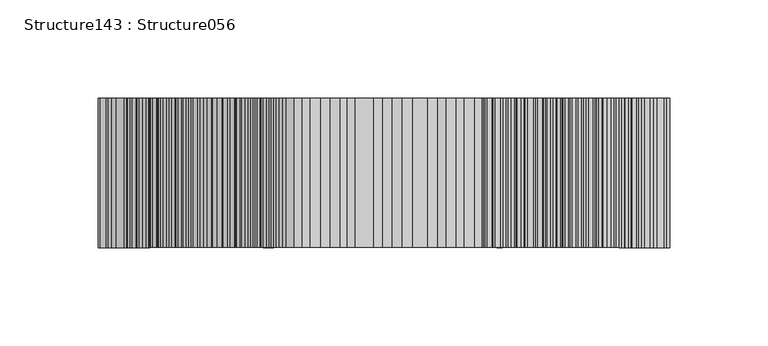
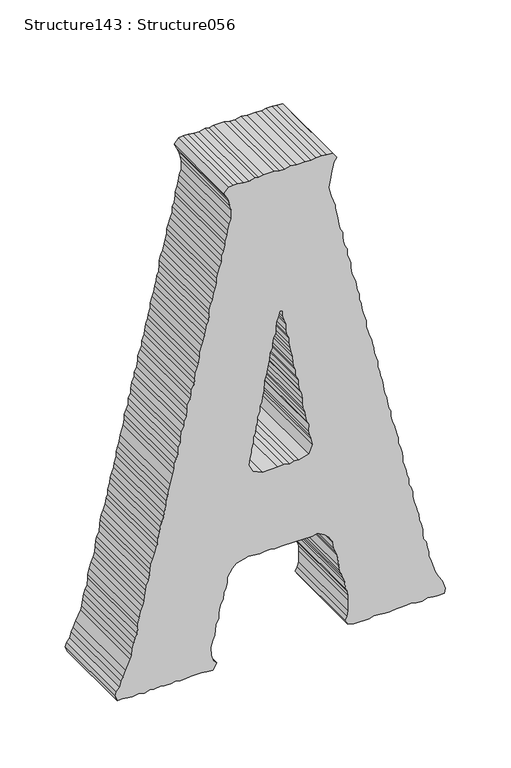
"""IFC4 building model written with IfcOpenShell, lengths in millimetres: proxy geometry, Structure143 : Structure056."""

from ifc_helpers import new_model, si_unit, frame, origin, place, context, project, spatial, polyline, outline, extrude, source, transform, mapped, element, save


def structure143_structure056_8a1e39fe(model_context):
    return source(origin(), model_context, "Body", "SweptSolid", [
        extrude(outline(polyline([(3818.8310229, -43679.9409523), (3814.7296538, -43679.9409523), (3811.2043377, -43681.1219412), (3805.9476534, -43683.4614546), (3801.8462843, -43683.4614546), (3795.960595, -43684.0631813), (3791.8865042, -43686.4026946), (3787.7867397, -43686.4026946), (3783.0868532, -43688.7438126), (3777.8285642, -43689.3230748), (3773.11905, -43689.3230748), (3769.6274306, -43691.6625882), (3763.759392, -43691.6625882), (3759.6596275, -43693.4228393), (3755.559863, -43695.184695), (3750.8583719, -43695.184695), (3746.1745313, -43696.3432195), (3737.400554, -43698.7051973), (3732.1149867, -43699.8861862), (3727.4311462, -43701.0447107), (3723.3313817, -43702.2273042), (3718.6571688, -43702.2273042), (3713.3555556, -43703.9650908), (3709.2718371, -43704.5443531), (3704.5879966, -43706.3270687), (3701.0723082, -43707.4855931), (3695.786741, -43708.0648553), (3690.512406, -43709.8267111), (3685.8285655, -43709.8267111), (3682.8857208, -43711.0077), (3677.6274319, -43712.1662244), (3672.9435914, -43713.9264755), (3668.8261762, -43715.6867267), (3664.1423357, -43716.2675935), (3660.0682449, -43716.8693202), (3654.1841602, -43717.4485824), (3650.1004418, -43719.7880958), (3645.9830266, -43720.367358), (3641.2991861, -43720.9690847), (3636.0408972, -43721.5483469), (3631.915459, -43722.7068713), (3627.8397636, -43724.4911915), (3622.555801, -43726.2289782), (3617.2718384, -43727.4099671), (3613.772196, -43727.4099671), (3607.8961343, -43727.9892293), (3604.3964919, -43729.7494805), (3600.2967274, -43730.9304694), (3595.5872132, -43732.0905984), (3589.7544759, -43732.6923251), (3586.2115092, -43733.8508496), (3577.4535778, -43737.9506141), (3572.1423369, -43740.291732), (3568.6426945, -43742.0519831), (3563.366755, -43743.2329721), (3560.441561, -43746.1533522), (3556.3417965, -43747.3343411), (3551.6675836, -43745.5724854), (3551.6675836, -43740.8934587), (3551.0658569, -43736.1903629), (3550.4833855, -43732.0905984), (3551.6675836, -43726.8307049), (3550.4833855, -43721.5483469), (3551.6675836, -43716.8693202), (3551.0658569, -43713.3472133), (3551.6675836, -43707.4855931), (3551.0658569, -43703.9650908), (3551.0658569, -43698.1034706), (3551.6675836, -43694.0037061), (3551.0658569, -43689.902337), (3551.0658569, -43685.2217057), (3551.6675836, -43680.542679), (3551.6675836, -43671.1589519), (3551.0658569, -43666.4799252), (3550.4833855, -43661.1975672), (3556.3417965, -43657.6770649), (3559.2669905, -43660.618305), (3565.1254015, -43662.3785561), (3572.7440636, -43662.9578183), (3578.6104977, -43661.1975672), (3582.7102621, -43659.4373161), (3587.3860796, -43658.8580539), (3592.0955938, -43658.2787916), (3596.7698067, -43655.9152092), (3601.4536473, -43655.9152092), (3604.9709403, -43655.335947), (3610.2292293, -43654.1774225), (3613.772196, -43651.8154447), (3619.6145609, -43651.2361825), (3622.555801, -43649.4759314), (3627.8397636, -43648.3158023), (3633.0980525, -43648.3158023), (3639.5405396, -43643.6367756), (3643.0578326, -43640.0922043), (3644.8245022, -43633.0720596), (3645.9830266, -43629.5515573), (3645.4262289, -43623.7124016), (3644.8245022, -43619.5901726), (3645.4262289, -43614.9095413), (3645.9830266, -43610.22891), (3644.8245022, -43606.1291455), (3645.4262289, -43600.8467875), (3645.4262289, -43588.5442849), (3644.8245022, -43582.6842692), (3644.8245022, -43573.3005421), (3645.9830266, -43568.6215154), (3642.4833842, -43562.180633), (3638.9580681, -43558.0792639), (3633.0980525, -43555.1380239), (3627.2396415, -43553.9794994), (3622.555801, -43552.2176437), (3619.6145609, -43551.0366548), (3609.0723094, -43549.8781303), (3604.3964919, -43548.6971414), (3600.2967274, -43547.538617), (3596.1953583, -43545.7783658), (3592.0955938, -43544.5957723), (3586.2115092, -43544.0165101), (3582.7102621, -43542.256259), (3578.6104977, -43541.0977345), (3573.9266571, -43541.0977345), (3563.9412034, -43541.0977345), (3559.2669905, -43542.256259), (3555.7416744, -43544.0165101), (3551.6675836, -43541.6769967), (3550.4833855, -43536.3946387), (3550.4833855, -43522.9336116), (3551.6675836, -43518.8338471), (3551.0658569, -43513.5514891), (3550.4833855, -43508.849998), (3550.4833855, -43504.7710933), (3551.0658569, -43498.8870087), (3551.0658569, -43494.7872442), (3551.6675836, -43490.1066129), (3551.6675836, -43486.0068484), (3550.4833855, -43481.3262171), (3550.4833855, -43476.0438591), (3551.6675836, -43471.3648324), (3551.0658569, -43466.0824744), (3550.4833855, -43462.5828319), (3551.0658569, -43456.7003519), (3555.1848766, -43455.5402228), (3560.441561, -43457.3020786), (3563.366755, -43458.460603), (3568.6426945, -43461.9811053), (3572.1423369, -43463.742961), (3576.2693797, -43465.5032121), (3586.2115092, -43468.4219877), (3590.3289243, -43470.1822388), (3594.4286888, -43470.1822388), (3599.1125293, -43471.3648324), (3604.3964919, -43472.5233568), (3608.4705827, -43474.8853346), (3612.5976255, -43475.4645968), (3617.2718384, -43475.4645968), (3622.555801, -43476.6231213), (3627.2396415, -43478.4058369), (3632.5155811, -43478.9642392), (3636.0408972, -43480.1452282), (3640.114988, -43481.3262171), (3645.4262289, -43483.0640037), (3650.6845178, -43484.2449926), (3655.3587307, -43484.2449926), (3659.4584952, -43485.4259815), (3663.5598643, -43487.7670995), (3668.8261762, -43487.7670995), (3673.5276674, -43489.5273506), (3677.0449604, -43490.1066129), (3682.8857208, -43491.866864), (3686.4030139, -43493.0478529), (3691.0868544, -43493.0478529), (3695.2122926, -43493.6287197), (3699.8881101, -43494.7872442), (3705.7545441, -43497.149222), (3710.4560353, -43497.149222), (3714.5301261, -43498.3077464), (3718.0554422, -43499.4887353), (3723.3313817, -43500.6697243), (3727.4311462, -43502.4091155), (3732.7167134, -43503.5901044), (3737.9750024, -43503.5901044), (3740.9162424, -43505.3503556), (3745.6000829, -43506.50888), (3751.4424479, -43507.1106067), (3756.1423345, -43508.849998), (3759.6596275, -43510.0309869), (3764.3611187, -43510.6102491), (3769.0176809, -43511.2119758), (3774.3032481, -43512.9497625), (3777.8285642, -43513.5514891), (3783.0868532, -43515.3117403), (3788.3611881, -43515.3117403), (3791.8865042, -43516.4718693), (3797.1463977, -43518.2321205), (3801.8462843, -43518.8338471), (3806.5317294, -43519.9923716), (3810.0474179, -43520.5716338), (3815.3313805, -43522.9336116), (3820.015221, -43524.0937407), (3824.1149855, -43525.2747296), (3829.374879, -43525.2747296), (3837.6000817, -43528.1935052), (3842.8583706, -43529.3744941), (3846.9757858, -43529.9537563), (3851.6612309, -43531.715612), (3856.9179152, -43531.715612), (3861.0192843, -43533.4758632), (3866.3032469, -43534.0551254), (3869.8189354, -43534.6343876), (3873.9203044, -43536.3946387), (3878.5784713, -43538.1564945), (3883.8881076, -43539.3150189), (3888.5623205, -43539.3150189), (3892.6636896, -43540.4960078), (3897.3475301, -43542.256259), (3902.6314927, -43542.256259), (3906.1487857, -43544.5957723), (3910.8310217, -43545.7783658), (3916.0909152, -43546.3576281), (3919.6066036, -43546.3576281), (3924.2888396, -43548.6971414), (3928.9919353, -43549.8781303), (3934.2758979, -43550.4573925), (3938.9517154, -43551.6383815), (3944.235678, -43552.7985105), (3947.1496398, -43552.7985105), (3956.5349715, -43556.3190128), (3961.794865, -43557.5000017), (3965.8930249, -43558.6585261), (3974.7055128, -43556.898275), (3979.9621971, -43555.7397505), (3983.4794902, -43555.1380239), (3987.5792547, -43553.9794994), (3991.6806238, -43551.6383815), (3996.390138, -43555.1380239), (3996.9645864, -43560.4203819), (3997.5486624, -43564.5201463), (3997.5486624, -43569.8025043), (3996.390138, -43573.9022688), (3996.9645864, -43579.1846268), (3996.9645864, -43586.7840337), (3997.5486624, -43592.0663917), (3996.390138, -43597.3262853), (3996.390138, -43602.0277764), (3997.5486624, -43606.7084077), (3997.5486624, -43616.0905302), (3996.9645864, -43620.1918993), (3997.5486624, -43623.7124016), (3996.390138, -43628.9722951), (3996.390138, -43633.6513218), (3997.5486624, -43638.9336798), (3997.5486624, -43643.0350489), (3996.9645864, -43647.1348134), (3992.2614906, -43651.2361825), (3987.5792547, -43648.8950645), (3984.0635662, -43647.1348134), (3979.3781211, -43645.976289), (3974.7055128, -43644.7953001), (3966.5043792, -43644.7953001), (3962.3757319, -43646.5555512), (3957.1190475, -43647.7140756), (3952.435207, -43648.3158023), (3947.7337158, -43650.0776581), (3944.235678, -43650.0776581), (3938.3499888, -43651.2361825), (3934.8503464, -43652.9964336), (3929.5904528, -43652.9964336), (3924.8905662, -43654.7566848), (3919.6066036, -43656.5169359), (3915.5068392, -43657.6770649), (3910.8310217, -43657.6770649), (3906.1487857, -43658.8580539), (3902.6314927, -43660.0165783), (3896.763454, -43661.1975672), (3893.822214, -43662.9578183), (3888.5623205, -43664.1388073), (3884.4609514, -43664.1388073), (3878.5784713, -43664.7196741), (3875.0772243, -43666.4799252), (3870.4030114, -43667.0591874), (3866.3032469, -43668.2401763), (3861.0192843, -43669.3987008), (3856.9179152, -43670.5796897), (3851.6612309, -43672.3415454), (3846.9757858, -43672.3415454), (3841.6741725, -43674.0793321), (3838.1761347, -43674.6810588), (3833.4730389, -43676.4413099), (3828.2163546, -43677.0205721), (3824.1149855, -43677.5998344), (3818.8310229, -43679.9409523)]), holes=[polyline([(3720.4158154, -43617.2490547), (3723.9154578, -43625.4501883), (3730.9323932, -43628.9722951), (3736.7988273, -43627.8137707), (3741.5003184, -43626.6311772), (3744.9999608, -43626.6311772), (3750.3015741, -43624.870926), (3755.559863, -43624.870926), (3759.0595054, -43623.1106749), (3764.3611187, -43622.5314127), (3768.4432325, -43621.3504238), (3773.11905, -43621.3504238), (3777.8285642, -43619.0093058), (3783.0868532, -43619.0093058), (3786.0280932, -43617.2490547), (3790.7039107, -43616.6697925), (3795.4037973, -43615.4888035), (3804.7730829, -43614.9095413), (3810.0474179, -43613.1492902), (3814.7296538, -43612.570028), (3818.8310229, -43611.3874345), (3822.932392, -43610.8081722), (3828.790803, -43610.22891), (3833.4730389, -43607.8893967), (3836.9919366, -43607.8893967), (3842.2758992, -43607.28767), (3845.8012153, -43604.9481566), (3851.0595042, -43604.9481566), (3855.7353217, -43604.3672898), (3860.4432313, -43602.6070387), (3865.1190488, -43601.4485142), (3864.5446004, -43599.6657986), (3860.4432313, -43599.6657986), (3856.3161885, -43598.5072742), (3851.6612309, -43596.7454184), (3846.3772683, -43596.7454184), (3842.2758992, -43596.1661562), (3837.6000817, -43593.8266429), (3832.8921721, -43593.8266429), (3828.790803, -43593.2249162), (3824.1149855, -43592.0663917), (3819.4150989, -43590.8854028), (3813.5743386, -43590.3061406), (3810.0474179, -43589.7252738), (3805.9476534, -43587.9650226), (3800.6717138, -43587.9650226), (3795.4037973, -43585.6255093), (3790.7039107, -43585.6255093), (3786.0280932, -43584.4445204), (3782.5027771, -43582.6842692), (3777.2444882, -43582.1034024), (3772.5606477, -43582.1034024), (3767.8607611, -43581.5016757), (3763.759392, -43579.7638891), (3759.6596275, -43579.1846268), (3754.9854146, -43578.5829001), (3750.8583719, -43576.2433868), (3744.9999608, -43576.822649), (3740.9162424, -43575.6641246), (3736.7988273, -43574.4815311), (3730.9323932, -43573.3005421), (3723.3313817, -43576.2433868), (3720.4158154, -43585.0237826), (3720.9726131, -43589.1235471), (3719.8140887, -43593.2249162), (3720.9726131, -43598.5072742), (3720.4158154, -43603.7880276), (3720.4158154, -43617.2490547)])]), frame((0.0, 247945.1599557, 0.0), z_axis=(0.0, 1.0, 0.0), x_axis=(0.0, 0.0, 1.0)), (0.0, 0.0, 1.0), 76.2),
    ])


if __name__ == "__main__":
    model = new_model("IFC4")
    model_context = context("Model", 3, world=origin())
    ifc_project = project(units=[si_unit("LENGTHUNIT", "METRE", prefix="MILLI")], contexts=[model_context])
    site = spatial("IfcSite", under=ifc_project)
    building = spatial("IfcBuilding", under=site)
    placement = place(None, origin())
    structure143_structure056_shape = structure143_structure056_8a1e39fe(model_context)
    element("IfcBuildingElementProxy", 1, Name="Structure143 : Structure056", ObjectType="Structure143 : Structure056", at=placement, inside=building, context=model_context, shape_type="MappedRepresentation", body=[
        mapped(structure143_structure056_shape, transform((0.0, 0.0, 0.0), x_axis=(1.0, 0.0, 0.0), y_axis=(0.0, 1.0, 0.0), z_axis=(0.0, 0.0, 1.0))),
    ])
    save(model, "model.ifc")

# Revit data of these elements
# Type "Structure143 : Structure056"
#   NameOverride = "Structure056"
# Element 1 (IfcBuildingElementProxy, "Structure143 : Structure056")
#   Materials on its faces: "BRUSHED ALUM. LETTERING"
# Materials
#   "BRUSHED ALUM. LETTERING": class "Unassigned", colour RGB 169 181 186, transparency 0, Cost = 0
